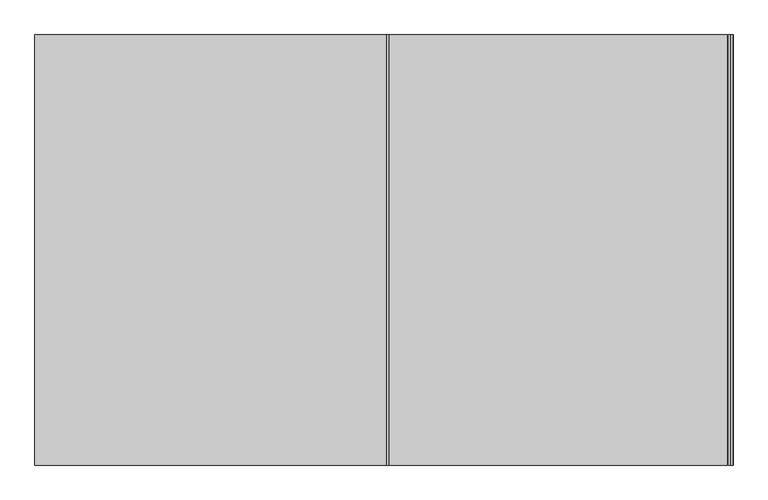
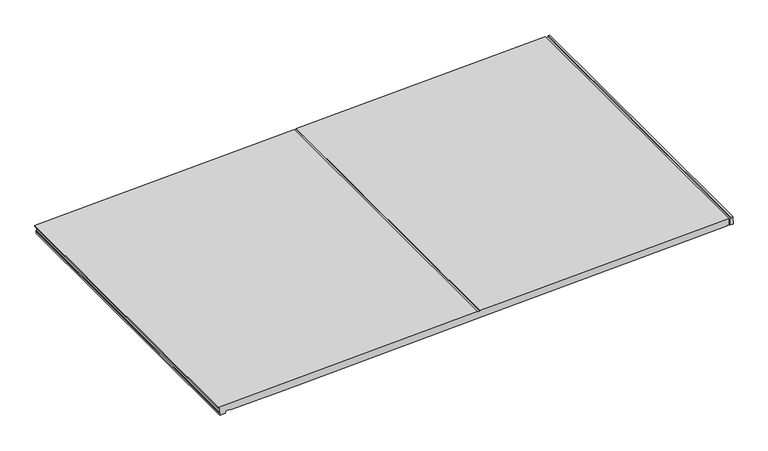
"""IFC4 building model written with IfcOpenShell, lengths in millimetres: proxy geometry, Generic Models 7:Generic Models 1:337419:Generic Models 1:337419 : Generic Models 7:Generic Models 1:337419:37 : Generic Models 7:Generic Models 1:337419:Generic Models 1:337419 : Generic Models 7:Generic Models 1:337419:301336."""

from ifc_helpers import new_model, si_unit, origin, place, context, project, spatial, faceted_brep, source, transform, mapped, element, save


def generic_models_6b6318d3(model_context):
    return source(origin(), model_context, "Body", "Brep", [
        faceted_brep([(560595.6172896, -567197.5812453, 3679.8374038), (560570.6490415, -567197.5812453, 3678.7970601), (560570.6490415, -567197.5812453, 3615.394447), (560364.5683367, -567197.5812453, 3615.394447), (560364.5683367, -567197.5812453, 3717.3710203), (560333.9392488, -567197.5812453, 3716.0948083), (560333.7860389, -567197.5812453, 3719.7718464), (560374.3804831, -567197.5812453, 3721.4632816), (560374.3804831, -567197.5812453, 3912.1285745), (560310.0813364, -567197.5812453, 3909.4494434), (560308.4952127, -567197.5812453, 3947.5164135), (569786.7341423, -567197.5812453, 4342.4430355), (569787.7915582, -567197.5812453, 4317.0650555), (569873.2872899, -567197.5812453, 4320.6273776), (569872.2298741, -567197.5812453, 4346.0053577), (578979.6356222, -567197.5812453, 4725.4805972), (578979.6356222, -567197.5812453, 4468.3138619), (578916.1356222, -567197.5812453, 4468.3138619), (578916.1356222, -567197.5812453, 4443.1923343), (560760.3165945, -567197.5812453, 3686.6998748), (560759.1534371, -567197.5812453, 3714.6156529), (560594.4541322, -567197.5812453, 3707.7531819), (560595.6172896, -578800.666382, 3679.8374038), (560594.4541322, -578800.666382, 3707.7531819), (560759.1534371, -578800.666382, 3714.6156529), (560760.3165945, -578800.666382, 3686.6998748), (562721.2246473, -578800.666382, 3768.404377), (570490.7367239, -578800.666382, 4092.1340469), (578916.1356222, -578800.666382, 4443.1923343), (578916.1356222, -578800.666382, 4468.3138619), (578979.6356222, -578800.666382, 4468.3138619), (578979.6356222, -578800.666382, 4725.4805972), (570490.7367239, -578800.666382, 4371.7764764), (569872.2298741, -578800.666382, 4346.0053577), (569873.2872899, -578800.666382, 4320.6273776), (569787.7915582, -578800.666382, 4317.0650555), (569786.7341423, -578800.666382, 4342.4430355), (560859.6126799, -578800.666382, 3970.4796413), (560308.4952127, -578800.666382, 3947.5164135), (560310.0813364, -578800.666382, 3909.4494434), (560374.3804831, -578800.666382, 3912.1285745), (560374.3804831, -578800.666382, 3721.4632816), (560333.7860389, -578800.666382, 3719.7718464), (560333.9392488, -578800.666382, 3716.0948083), (560364.5683367, -578800.666382, 3717.3710203), (560364.5683367, -578800.666382, 3615.394447), (560570.6490415, -578800.666382, 3615.394447), (560570.6490415, -578800.666382, 3678.7970601), (569786.7341423, -578799.0788841, 4342.4430355), (569787.7915582, -578799.0788841, 4317.0650555), (569873.2872899, -578799.0788841, 4320.6273776), (569872.2298741, -578799.0788841, 4346.0053577)], [[[0, 1, 2, 3, 4, 5, 6, 7, 8, 9, 10, 11, 12, 13, 14, 15, 16, 17, 18, 19, 20, 21]], [[22, 23, 24, 25, 26, 27, 28, 29, 30, 31, 32, 33, 34, 35, 36, 37, 38, 39, 40, 41, 42, 43, 44, 45, 46, 47]], [[1, 0, 22, 47]], [[9, 8, 40, 39]], [[10, 9, 39, 38]], [[11, 10, 38, 37, 36, 48]], [[12, 11, 48, 36, 35, 49]], [[13, 12, 49, 35, 34, 50]], [[14, 13, 50, 34, 33, 51]], [[19, 18, 28, 27, 26, 25]], [[20, 19, 25, 24]], [[21, 20, 24, 23]], [[0, 21, 23, 22]], [[2, 1, 47, 46]], [[3, 2, 46, 45]], [[4, 3, 45, 44]], [[5, 4, 44, 43]], [[6, 5, 43, 42]], [[7, 6, 42, 41]], [[8, 7, 41, 40]], [[15, 14, 51, 33, 32, 31]], [[16, 15, 31, 30]], [[17, 16, 30, 29]], [[18, 17, 29, 28]]]),
        faceted_brep([(579132.3000335, -567197.5812453, 4731.8416143), (579143.9316077, -567197.5812453, 4452.6838337), (579014.7791177, -567197.5812453, 4447.30248), (579014.7791177, -567197.5812453, 4667.6798093), (579077.31441, -567197.5812453, 4678.7064686), (579075.1995784, -567197.5812453, 4729.4624287), (579132.3000335, -578800.666382, 4731.8416143), (579075.1995784, -578800.666382, 4729.4624287), (579077.31441, -578800.666382, 4678.7064686), (579014.7791177, -578800.666382, 4667.6798093), (579014.7791177, -578800.666382, 4447.30248), (579143.9316077, -578800.666382, 4452.6838337), (579132.3000335, -578797.4913841, 4731.8416143), (579132.3000335, -573942.9163841, 4731.8416143), (579143.9316077, -578797.4913841, 4452.6838337), (579143.9316077, -573942.9163841, 4452.6838337)], [[[0, 1, 2, 3, 4, 5]], [[6, 7, 8, 9, 10, 11]], [[0, 5, 7, 6, 12, 13]], [[1, 0, 13, 12, 6, 11, 14, 15]], [[2, 1, 15, 14, 11, 10]], [[3, 2, 10, 9]], [[4, 3, 9, 8]], [[5, 4, 8, 7]]]),
    ])


if __name__ == "__main__":
    model = new_model("IFC4")
    model_context = context("Model", 3, world=origin())
    ifc_project = project(units=[si_unit("LENGTHUNIT", "METRE", prefix="MILLI")], contexts=[model_context])
    site = spatial("IfcSite", under=ifc_project)
    building = spatial("IfcBuilding", under=site)
    placement = place(None, origin())
    generic_models_shape = generic_models_6b6318d3(model_context)
    element("IfcBuildingElementProxy", 1, Name="Generic Models 7:Generic Models 1:337419:Generic Models 1:337419 : Generic Models 7:Generic Models 1:337419:37 : Generic Models 7:Generic Models 1:337419:Generic Models 1:337419 : Generic Models 7:Generic Models 1:337419:301336", ObjectType="Generic Models 7:Generic Models 1:337419:Generic Models 1:337419 : Generic Models 7:Generic Models 1:337419:37 : Generic Models 7:Generic Models 1:337419:Generic Models 1:337419 : Generic Models 7:Generic Models 1:337419:301336", at=placement, inside=building, context=model_context, shape_type="MappedRepresentation", body=[
        mapped(generic_models_shape, transform((0.0, 0.0, 0.0), x_axis=(1.0, 0.0, 0.0), y_axis=(0.0, 1.0, 0.0), z_axis=(0.0, 0.0, 1.0))),
    ])
    save(model, "model.ifc")

# Revit data of these elements
# Type "Generic Models 7:Generic Models 1:337419:Generic Models 1:337419 : Generic Models 7:Generic Models 1:337419:37 : Generic Models 7:Generic Models 1:337419:Generic Models 1:337419 : Generic Models 7:Generic Models 1:337419:301336"
#   NameOverride = "Generic Models 7:Generic Models 1:337419:Generic Models 1:337419 : Generic Models 7:Generic Models 1:337419:301336"
#   ObjectTypeOverride = "Generic Models 1:337419 : Generic Models 7:Generic Models 1:337419"
#   Reference = "Generic Models 1"
#   Tag = "301336"
# Element 1 (IfcBuildingElementProxy, "Generic Models 7:Generic Models 1:337419:Generic Models 1:337419 : Generic Models 7:Generic Models 1:337419:37 : Generic Models 7:Generic Models 1:337419:Generic Models 1:337419 : Generic Models 7:Generic Models 1:337419:301336")
#   Materials on its faces: "FULL CAVITY CLASS A FIBERGLASS INSULATION WITH DURABLE VAPOR BARRIER (BLACK) LINER"
# Materials
#   "FULL CAVITY CLASS A FIBERGLASS INSULATION WITH DURABLE VAPOR BARRIER (BLACK) LINER": class "Unassigned", colour RGB 158 92 175, transparency 0, Cost = 0
